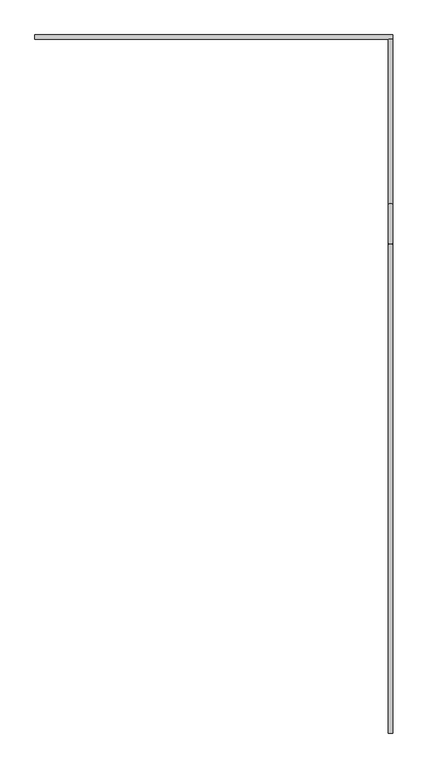
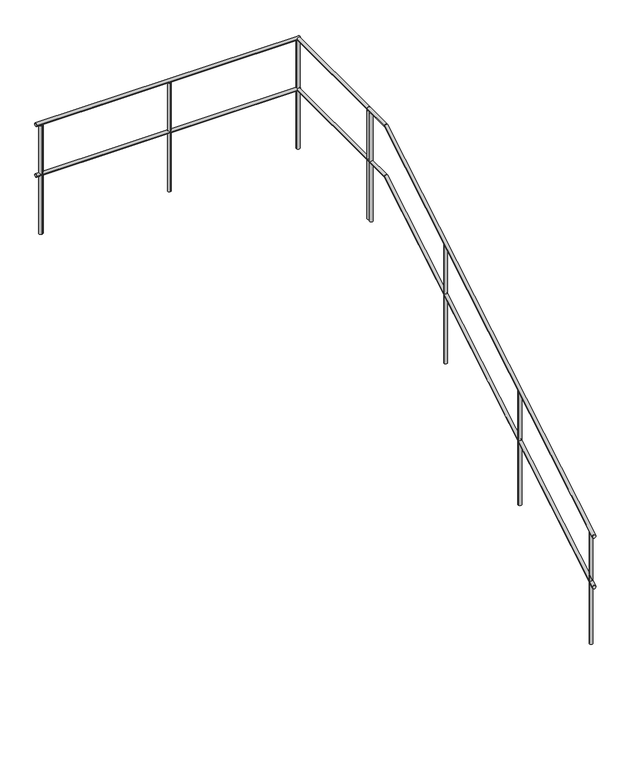
"""IFC4 building model written with IfcOpenShell, lengths in millimetres: railing geometry."""

from ifc_helpers import new_model, si_unit, point, frame, frame_2d, origin, place, context, project, spatial, circle_curve, ellipse_curve, trimmed, segment, composite_curve, outline, extrude, source, transform, mapped, element, save
from ifc_brep_helpers import plane_surface, cylinder_surface, advanced_brep


def railing_9a6f80a0(model_context):
    return source(origin(), model_context, "Body", "SolidModel", [
        advanced_brep(
        [(12685.1052251, 14699.5208589, 749.8338893), (12655.1052251, 14699.5208589, 749.8338893), (12685.1052251, 18339.5208589, 2760.0), (12655.1052251, 18339.5208589, 2760.0), (12685.1052251, 18063.6609247, 2760.0), (12655.1052251, 18063.6609247, 2760.0)],
        [
            (0, 1, ellipse_curve(frame((12670.1052251, 14699.5208589, 749.8338893), z_axis=(0.0, -1.0, 0.0), x_axis=(0.0, 0.0, -1.0)), 17.4738031, 15.0)),
            (1, 0, ellipse_curve(frame((12670.1052251, 14699.5208589, 749.8338893), z_axis=(0.0, -1.0, 0.0), x_axis=(0.0, 0.0, -1.0)), 17.4738031, 15.0)),
            (2, 3, circle_curve(frame((12670.1052251, 18339.5208589, 2760.0), z_axis=(0.0, 1.0, 0.0), x_axis=(-1.0, 0.0, 0.0)), 15.0)),
            (3, 2, circle_curve(frame((12670.1052251, 18339.5208589, 2760.0), z_axis=(0.0, 1.0, 0.0), x_axis=(-1.0, 0.0, 0.0)), 15.0)),
            (0, 4),
            (4, 5, ellipse_curve(frame((12670.1052251, 18063.6609247, 2760.0), z_axis=(0.0, -0.9639574411334471, -0.2660564821301241), x_axis=(0.0, 0.2660564821301243, -0.9639574411334468)), 15.560853, 15.0)),
            (5, 1),
            (5, 4, ellipse_curve(frame((12670.1052251, 18063.6609247, 2760.0), z_axis=(0.0, -0.9639574411334471, -0.2660564821301241), x_axis=(0.0, 0.2660564821301243, -0.9639574411334468)), 15.560853, 15.0)),
            (4, 2),
            (3, 5),
        ],
        [
            plane_surface(frame((12670.1052251, 14699.5208589, 767.3076923), z_axis=(0.0, -1.0, 0.0), x_axis=(0.0, 0.0, 1.0))),
            plane_surface(frame((12670.1052251, 18339.5208589, 2775.0), z_axis=(0.0, 1.0, 0.0), x_axis=(0.0, 0.0, 1.0))),
            cylinder_surface(frame((12670.1052251, 14707.2148727, 754.4312739), z_axis=(0.0, -0.8584278966330859, -0.5129342514222421), x_axis=(-1.0, 0.0, 0.0)), 15.0),
            cylinder_surface(frame((12670.1052251, 18059.5208589, 2760.0), z_axis=(0.0, -1.0, 0.0), x_axis=(-1.0, 0.0, 0.0)), 15.0),
        ],
        [
            (0, [[1, 2]]),
            (1, [[3, 4]]),
            (2, [[-1, 5, 6, 7]]),
            (2, [[-2, -7, 8, -5]]),
            (3, [[-6, 9, -4, 10]]),
            (3, [[-8, -10, -3, -9]]),
        ],
    ),
        advanced_brep(
        [(12685.1052251, 18339.5208589, 2760.0), (12655.1052251, 18339.5208589, 2760.0), (12685.1052251, 19469.5208589, 2760.0), (12655.1052251, 19469.5208589, 2760.0)],
        [
            (0, 1, circle_curve(frame((12670.1052251, 18339.5208589, 2760.0), z_axis=(0.0, -1.0, 0.0), x_axis=(-1.0, 0.0, 0.0)), 15.0)),
            (1, 0, circle_curve(frame((12670.1052251, 18339.5208589, 2760.0), z_axis=(0.0, -1.0, 0.0), x_axis=(-1.0, 0.0, 0.0)), 15.0)),
            (2, 3, circle_curve(frame((12670.1052251, 19469.5208589, 2760.0), z_axis=(0.0, 1.0, 0.0), x_axis=(-1.0, 0.0, 0.0)), 15.0)),
            (3, 2, circle_curve(frame((12670.1052251, 19469.5208589, 2760.0), z_axis=(0.0, 1.0, 0.0), x_axis=(-1.0, 0.0, 0.0)), 15.0)),
            (0, 2),
            (3, 1),
        ],
        [
            plane_surface(frame((12670.1052251, 18339.5208589, 2775.0), z_axis=(0.0, -1.0, 0.0), x_axis=(0.0, 0.0, 1.0))),
            plane_surface(frame((12670.1052251, 19469.5208589, 2775.0), z_axis=(0.0, 1.0, 0.0), x_axis=(0.0, 0.0, 1.0))),
            cylinder_surface(frame((12670.1052251, 18339.5208589, 2760.0), z_axis=(0.0, -1.0, 0.0), x_axis=(-1.0, 0.0, 0.0)), 15.0),
        ],
        [
            (0, [[1, 2]]),
            (1, [[3, 4]]),
            (2, [[-1, 5, -4, 6]]),
            (2, [[-2, -6, -3, -5]]),
        ],
    ),
        advanced_brep(
        [(12685.1052251, 19499.5208589, 2760.0), (12685.1052251, 19469.5208589, 2760.0), (10225.1052251, 19499.5208589, 2760.0), (10225.1052251, 19469.5208589, 2760.0)],
        [
            (0, 1, circle_curve(frame((12685.1052251, 19484.5208589, 2760.0), z_axis=(1.0, 0.0, 0.0), x_axis=(0.0, -1.0, 0.0)), 15.0)),
            (1, 0, circle_curve(frame((12685.1052251, 19484.5208589, 2760.0), z_axis=(1.0, 0.0, 0.0), x_axis=(0.0, -1.0, 0.0)), 15.0)),
            (2, 3, circle_curve(frame((10225.1052251, 19484.5208589, 2760.0), z_axis=(-1.0, 0.0, 0.0), x_axis=(0.0, -1.0, 0.0)), 15.0)),
            (3, 2, circle_curve(frame((10225.1052251, 19484.5208589, 2760.0), z_axis=(-1.0, 0.0, 0.0), x_axis=(0.0, -1.0, 0.0)), 15.0)),
            (0, 2),
            (3, 1),
        ],
        [
            plane_surface(frame((12685.1052251, 19484.5208589, 2775.0), z_axis=(1.0, 0.0, 0.0), x_axis=(0.0, -1.0, 0.0))),
            plane_surface(frame((10225.1052251, 19484.5208589, 2775.0), z_axis=(-1.0, 0.0, 0.0), x_axis=(0.0, -1.0, 0.0))),
            cylinder_surface(frame((12685.1052251, 19484.5208589, 2760.0), z_axis=(1.0, 0.0, 0.0), x_axis=(0.0, -1.0, 0.0)), 15.0),
        ],
        [
            (0, [[1, 2]]),
            (1, [[3, 4]]),
            (2, [[-1, 5, -4, 6]]),
            (2, [[-2, -6, -3, -5]]),
        ],
    ),
        advanced_brep(
        [(12685.1052251, 14699.5208589, 1249.8338893), (12655.1052251, 14699.5208589, 1249.8338893), (12685.1052251, 18063.6609247, 3260.0), (12655.1052251, 18063.6609247, 3260.0), (12685.1052251, 18339.5208589, 3260.0), (12655.1052251, 18339.5208589, 3260.0)],
        [
            (0, 1, ellipse_curve(frame((12670.1052251, 14699.5208589, 1249.8338893), z_axis=(0.0, -1.0, 0.0), x_axis=(0.0, 0.0, -1.0)), 17.4738031, 15.0)),
            (1, 0, ellipse_curve(frame((12670.1052251, 14699.5208589, 1249.8338893), z_axis=(0.0, -1.0, 0.0), x_axis=(0.0, 0.0, -1.0)), 17.4738031, 15.0)),
            (0, 2),
            (2, 3, ellipse_curve(frame((12670.1052251, 18063.6609247, 3260.0), z_axis=(0.0, -0.9639574411334471, -0.2660564821301241), x_axis=(0.0, 0.2660564821301243, -0.9639574411334468)), 15.560853, 15.0)),
            (3, 1),
            (3, 2, ellipse_curve(frame((12670.1052251, 18063.6609247, 3260.0), z_axis=(0.0, -0.9639574411334471, -0.2660564821301241), x_axis=(0.0, 0.2660564821301243, -0.9639574411334468)), 15.560853, 15.0)),
            (4, 5, circle_curve(frame((12670.1052251, 18339.5208589, 3260.0), z_axis=(0.0, 1.0, 0.0), x_axis=(-1.0, 0.0, 0.0)), 15.0)),
            (5, 4, circle_curve(frame((12670.1052251, 18339.5208589, 3260.0), z_axis=(0.0, 1.0, 0.0), x_axis=(-1.0, 0.0, 0.0)), 15.0)),
            (2, 4),
            (5, 3),
        ],
        [
            plane_surface(frame((12670.1052251, 14699.5208589, 1267.3076923), z_axis=(0.0, -1.0, 0.0), x_axis=(0.0, 0.0, 1.0))),
            cylinder_surface(frame((12670.1052251, 14707.2148727, 1254.4312739), z_axis=(0.0, -0.8584278966330859, -0.5129342514222421), x_axis=(-1.0, 0.0, 0.0)), 15.0),
            plane_surface(frame((12670.1052251, 18339.5208589, 3275.0), z_axis=(0.0, 1.0, 0.0), x_axis=(0.0, 0.0, 1.0))),
            cylinder_surface(frame((12670.1052251, 18059.5208589, 3260.0), z_axis=(0.0, -1.0, 0.0), x_axis=(-1.0, 0.0, 0.0)), 15.0),
        ],
        [
            (0, [[1, 2]]),
            (1, [[-1, 3, 4, 5]]),
            (1, [[-2, -5, 6, -3]]),
            (2, [[7, 8]]),
            (3, [[-4, 9, -8, 10]]),
            (3, [[-6, -10, -7, -9]]),
        ],
    ),
        advanced_brep(
        [(12685.1052251, 18339.5208589, 3260.0), (12655.1052251, 18339.5208589, 3260.0), (12685.1052251, 19469.5208589, 3260.0), (12655.1052251, 19469.5208589, 3260.0)],
        [
            (0, 1, circle_curve(frame((12670.1052251, 18339.5208589, 3260.0), z_axis=(0.0, -1.0, 0.0), x_axis=(-1.0, 0.0, 0.0)), 15.0)),
            (1, 0, circle_curve(frame((12670.1052251, 18339.5208589, 3260.0), z_axis=(0.0, -1.0, 0.0), x_axis=(-1.0, 0.0, 0.0)), 15.0)),
            (2, 3, circle_curve(frame((12670.1052251, 19469.5208589, 3260.0), z_axis=(0.0, 1.0, 0.0), x_axis=(-1.0, 0.0, 0.0)), 15.0)),
            (3, 2, circle_curve(frame((12670.1052251, 19469.5208589, 3260.0), z_axis=(0.0, 1.0, 0.0), x_axis=(-1.0, 0.0, 0.0)), 15.0)),
            (0, 2),
            (3, 1),
        ],
        [
            plane_surface(frame((12670.1052251, 18339.5208589, 3275.0), z_axis=(0.0, -1.0, 0.0), x_axis=(0.0, 0.0, 1.0))),
            plane_surface(frame((12670.1052251, 19469.5208589, 3275.0), z_axis=(0.0, 1.0, 0.0), x_axis=(0.0, 0.0, 1.0))),
            cylinder_surface(frame((12670.1052251, 18339.5208589, 3260.0), z_axis=(0.0, -1.0, 0.0), x_axis=(-1.0, 0.0, 0.0)), 15.0),
        ],
        [
            (0, [[1, 2]]),
            (1, [[3, 4]]),
            (2, [[-1, 5, -4, 6]]),
            (2, [[-2, -6, -3, -5]]),
        ],
    ),
        advanced_brep(
        [(12685.1052251, 19499.5208589, 3260.0), (12685.1052251, 19469.5208589, 3260.0), (10225.1052251, 19499.5208589, 3260.0), (10225.1052251, 19469.5208589, 3260.0)],
        [
            (0, 1, circle_curve(frame((12685.1052251, 19484.5208589, 3260.0), z_axis=(1.0, 0.0, 0.0), x_axis=(0.0, -1.0, 0.0)), 15.0)),
            (1, 0, circle_curve(frame((12685.1052251, 19484.5208589, 3260.0), z_axis=(1.0, 0.0, 0.0), x_axis=(0.0, -1.0, 0.0)), 15.0)),
            (2, 3, circle_curve(frame((10225.1052251, 19484.5208589, 3260.0), z_axis=(-1.0, 0.0, 0.0), x_axis=(0.0, -1.0, 0.0)), 15.0)),
            (3, 2, circle_curve(frame((10225.1052251, 19484.5208589, 3260.0), z_axis=(-1.0, 0.0, 0.0), x_axis=(0.0, -1.0, 0.0)), 15.0)),
            (0, 2),
            (3, 1),
        ],
        [
            plane_surface(frame((12685.1052251, 19484.5208589, 3275.0), z_axis=(1.0, 0.0, 0.0), x_axis=(0.0, -1.0, 0.0))),
            plane_surface(frame((10225.1052251, 19484.5208589, 3275.0), z_axis=(-1.0, 0.0, 0.0), x_axis=(0.0, -1.0, 0.0))),
            cylinder_surface(frame((12685.1052251, 19484.5208589, 3260.0), z_axis=(1.0, 0.0, 0.0), x_axis=(0.0, -1.0, 0.0)), 15.0),
        ],
        [
            (0, [[1, 2]]),
            (1, [[3, 4]]),
            (2, [[-1, 5, -4, 6]]),
            (2, [[-2, -6, -3, -5]]),
        ],
    ),
        extrude(outline(composite_curve([segment(trimmed(circle_curve(frame_2d((10270.1052251, 19484.5208589)), 15.0), [point((10270.1052251, 19469.5208589))], [point((10270.1052251, 19499.5208589))], False, "CARTESIAN"), True, "CONTINUOUS"), segment(trimmed(circle_curve(frame_2d((10270.1052251, 19484.5208589)), 15.0), [point((10270.1052251, 19499.5208589))], [point((10270.1052251, 19469.5208589))], False, "CARTESIAN"), True, "CONTINUOUS")], self_intersect=False)), frame((0.0, 0.0, 2175.0), z_axis=(0.0, 0.0, 1.0), x_axis=(1.0, 0.0, 0.0)), (0.0, 0.0, 1.0), 1070.0),
        extrude(outline(composite_curve([segment(trimmed(circle_curve(frame_2d((11470.1052251, 19484.5208589)), 15.0), [point((11470.1052251, 19469.5208589))], [point((11470.1052251, 19499.5208589))], False, "CARTESIAN"), True, "CONTINUOUS"), segment(trimmed(circle_curve(frame_2d((11470.1052251, 19484.5208589)), 15.0), [point((11470.1052251, 19499.5208589))], [point((11470.1052251, 19469.5208589))], False, "CARTESIAN"), True, "CONTINUOUS")], self_intersect=False)), frame((0.0, 0.0, 2175.0), z_axis=(0.0, 0.0, 1.0), x_axis=(1.0, 0.0, 0.0)), (0.0, 0.0, 1.0), 1070.0),
        extrude(outline(composite_curve([segment(trimmed(circle_curve(frame_2d((12670.1052251, 18299.5208589)), 15.0), [point((12655.1052251, 18299.5208589))], [point((12685.1052251, 18299.5208589))], False, "CARTESIAN"), True, "CONTINUOUS"), segment(trimmed(circle_curve(frame_2d((12670.1052251, 18299.5208589)), 15.0), [point((12685.1052251, 18299.5208589))], [point((12655.1052251, 18299.5208589))], False, "CARTESIAN"), True, "CONTINUOUS")], self_intersect=False)), frame((0.0, 0.0, 2175.0), z_axis=(0.0, 0.0, 1.0), x_axis=(1.0, 0.0, 0.0)), (0.0, 0.0, 1.0), 1070.0),
        extrude(outline(composite_curve([segment(trimmed(circle_curve(frame_2d((12670.1052251, 17099.5208589)), 15.0), [point((12655.1052251, 17099.5208589))], [point((12685.1052251, 17099.5208589))], False, "CARTESIAN"), True, "CONTINUOUS"), segment(trimmed(circle_curve(frame_2d((12670.1052251, 17099.5208589)), 15.0), [point((12685.1052251, 17099.5208589))], [point((12655.1052251, 17099.5208589))], False, "CARTESIAN"), True, "CONTINUOUS")], self_intersect=False)), frame((0.0, 0.0, 1505.7692308), z_axis=(0.0, 0.0, 1.0), x_axis=(1.0, 0.0, 0.0)), (0.0, 0.0, 1.0), 1165.6043956),
        extrude(outline(composite_curve([segment(trimmed(circle_curve(frame_2d((12670.1052251, 15899.5208589)), 15.0), [point((12655.1052251, 15899.5208589))], [point((12685.1052251, 15899.5208589))], False, "CARTESIAN"), True, "CONTINUOUS"), segment(trimmed(circle_curve(frame_2d((12670.1052251, 15899.5208589)), 15.0), [point((12685.1052251, 15899.5208589))], [point((12655.1052251, 15899.5208589))], False, "CARTESIAN"), True, "CONTINUOUS")], self_intersect=False)), frame((0.0, 0.0, 836.5384615), z_axis=(0.0, 0.0, 1.0), x_axis=(1.0, 0.0, 0.0)), (0.0, 0.0, 1.0), 1117.8021978),
        extrude(outline(composite_curve([segment(trimmed(circle_curve(frame_2d((12670.1052251, 19484.5208589)), 15.0), [point((12655.1052251, 19484.5208589))], [point((12685.1052251, 19484.5208589))], False, "CARTESIAN"), True, "CONTINUOUS"), segment(trimmed(circle_curve(frame_2d((12670.1052251, 19484.5208589)), 15.0), [point((12685.1052251, 19484.5208589))], [point((12655.1052251, 19484.5208589))], False, "CARTESIAN"), True, "CONTINUOUS")], self_intersect=False)), frame((0.0, 0.0, 2175.0), z_axis=(0.0, 0.0, 1.0), x_axis=(1.0, 0.0, 0.0)), (0.0, 0.0, 1.0), 1070.0),
        extrude(outline(composite_curve([segment(trimmed(circle_curve(frame_2d((12670.1052251, 18339.5208589)), 15.0), [point((12655.1052251, 18339.5208589))], [point((12685.1052251, 18339.5208589))], False, "CARTESIAN"), True, "CONTINUOUS"), segment(trimmed(circle_curve(frame_2d((12670.1052251, 18339.5208589)), 15.0), [point((12685.1052251, 18339.5208589))], [point((12655.1052251, 18339.5208589))], False, "CARTESIAN"), True, "CONTINUOUS")], self_intersect=False)), frame((0.0, 0.0, 2175.0), z_axis=(0.0, 0.0, 1.0), x_axis=(1.0, 0.0, 0.0)), (0.0, 0.0, 1.0), 1070.0),
        extrude(outline(composite_curve([segment(trimmed(circle_curve(frame_2d((10275.1052251, 19484.5208589)), 15.0), [point((10275.1052251, 19469.5208589))], [point((10275.1052251, 19499.5208589))], False, "CARTESIAN"), True, "CONTINUOUS"), segment(trimmed(circle_curve(frame_2d((10275.1052251, 19484.5208589)), 15.0), [point((10275.1052251, 19499.5208589))], [point((10275.1052251, 19469.5208589))], False, "CARTESIAN"), True, "CONTINUOUS")], self_intersect=False)), frame((0.0, 0.0, 2175.0), z_axis=(0.0, 0.0, 1.0), x_axis=(1.0, 0.0, 0.0)), (0.0, 0.0, 1.0), 1070.0),
        extrude(outline(composite_curve([segment(trimmed(circle_curve(frame_2d((12670.1052251, 14749.5208589)), 15.0), [point((12655.1052251, 14749.5208589))], [point((12685.1052251, 14749.5208589))], False, "CARTESIAN"), True, "CONTINUOUS"), segment(trimmed(circle_curve(frame_2d((12670.1052251, 14749.5208589)), 15.0), [point((12685.1052251, 14749.5208589))], [point((12655.1052251, 14749.5208589))], False, "CARTESIAN"), True, "CONTINUOUS")], self_intersect=False)), frame((0.0, 0.0, 167.3076923), z_axis=(0.0, 0.0, 1.0), x_axis=(1.0, 0.0, 0.0)), (0.0, 0.0, 1.0), 1099.8763736),
    ])


if __name__ == "__main__":
    model = new_model("IFC4")
    model_context = context("Model", 3, world=origin())
    ifc_project = project(units=[si_unit("LENGTHUNIT", "METRE", prefix="MILLI")], contexts=[model_context])
    site = spatial("IfcSite", under=ifc_project)
    building = spatial("IfcBuilding", under=site)
    placement = place(None, origin())
    railing_shape = railing_9a6f80a0(model_context)
    element("IfcRailing", 1, at=placement, inside=building, context=model_context, shape_type="MappedRepresentation", body=[
        mapped(railing_shape, transform((0.0, 0.0, 0.0), x_axis=(1.0, 0.0, 0.0), y_axis=(0.0, 1.0, 0.0), z_axis=(0.0, 0.0, 1.0))),
    ])
    save(model, "model.ifc")
